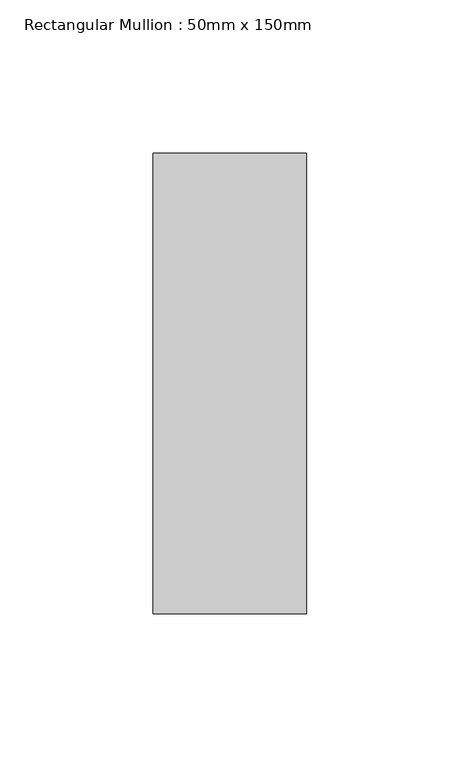
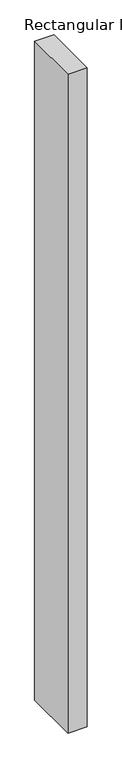
"""IFC4 building model written with IfcOpenShell, lengths in millimetres: member geometry, Rectangular Mullion : 50mm x 150mm."""

from ifc_helpers import new_model, si_unit, frame, origin, place, context, project, spatial, polyline, outline, extrude, source, transform, mapped, element, save


def rectangular_mullion_50mm_x_150mm_68ff1a14(model_context):
    return source(origin(), model_context, "Body", "SweptSolid", [
        extrude(outline(polyline([(0.0, 75.0), (0.0, -75.0), (-50.0, -75.0), (-50.0, 75.0), (0.0, 75.0)])), frame((0.0, 0.0, -1821.6686227), z_axis=(0.0, 0.0, 1.0), x_axis=(1.0, 0.0, 0.0)), (0.0, 0.0, 1.0), 1821.6686227),
    ])


if __name__ == "__main__":
    model = new_model("IFC4")
    model_context = context("Model", 3, world=origin())
    ifc_project = project(units=[si_unit("LENGTHUNIT", "METRE", prefix="MILLI")], contexts=[model_context])
    site = spatial("IfcSite", under=ifc_project)
    building = spatial("IfcBuilding", under=site)
    placement = place(None, origin())
    rectangular_mullion_50mm_x_150mm_shape = rectangular_mullion_50mm_x_150mm_68ff1a14(model_context)
    element("IfcMember", 1, ObjectType="Rectangular Mullion : 50mm x 150mm", at=placement, inside=building, context=model_context, shape_type="MappedRepresentation", body=[
        mapped(rectangular_mullion_50mm_x_150mm_shape, transform((0.0, 0.0, 0.0), x_axis=(1.0, 0.0, 0.0), y_axis=(0.0, 1.0, 0.0), z_axis=(0.0, 0.0, 1.0))),
    ])
    save(model, "model.ifc")

# Revit data of these elements
# Type "Rectangular Mullion : 50mm x 150mm"
#   built-in parameter 1007304 = 0.492126 (stored number, unit not read)
#   built-in parameter 1007301 = 0.082021 (stored number, unit not read)
#   built-in parameter 1007300 = 0.082021 (stored number, unit not read)
# Element 1 (IfcMember, "Rectangular Mullion : 50mm x 150mm")
#   Materials on its faces: "Aluminum"
# Materials
#   "Aluminum": class "Metal", colour RGB 244 244 244, transparency 0, Description = "Aluminum 6061", Cost = 0
